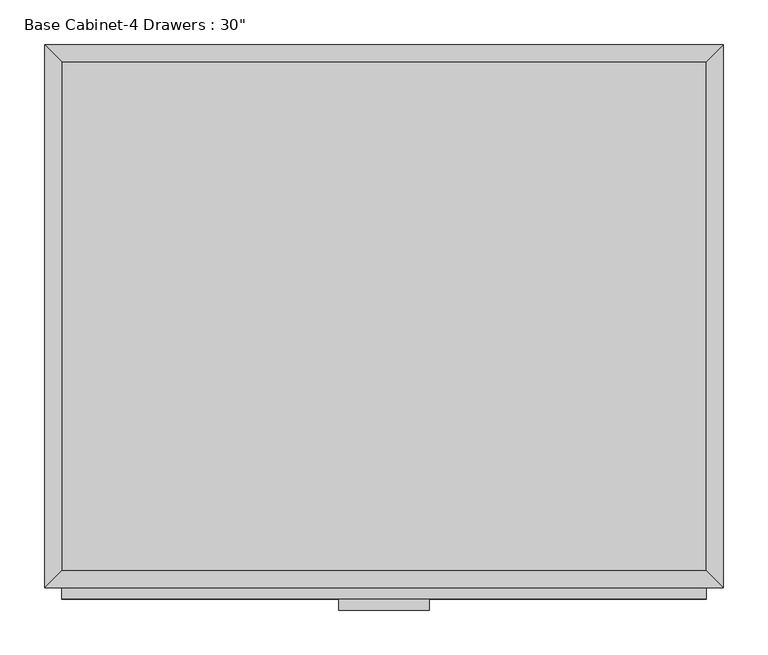
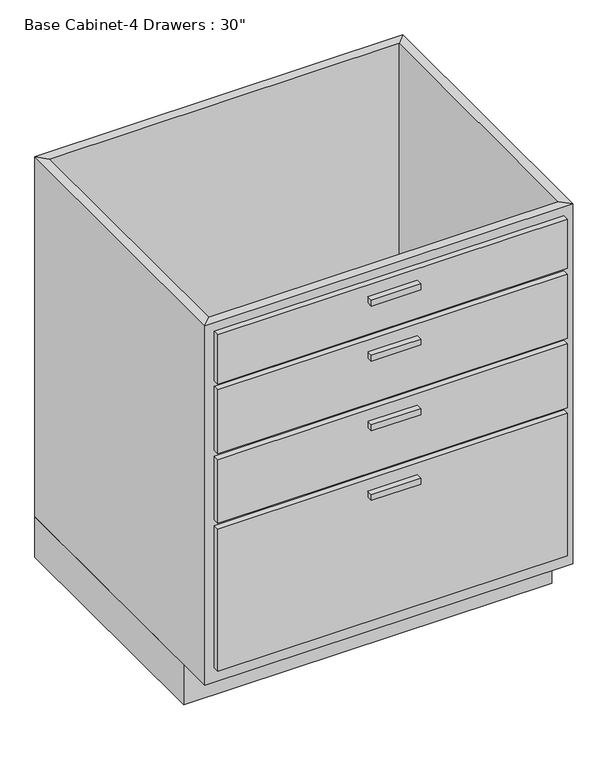
"""IFC4 building model written with IfcOpenShell, lengths in millimetres: furniture geometry."""

from ifc_helpers import new_model, si_unit, frame, origin, origin_with_axes, place, context, project, spatial, polyline, outline, extrude, faceted_brep, source, transform, mapped, element, save


def furniture_2c6c3b69(model_context):
    return source(origin(), model_context, "Body", "SolidModel", [
        extrude(outline(polyline([(69.5377049, -635.0), (-32.0622951, -635.0), (-32.0622951, -622.3), (69.5377049, -622.3), (69.5377049, -635.0)])), frame((0.0, 0.0, 819.15), z_axis=(0.0, 0.0, 1.0), x_axis=(1.0, 0.0, 0.0)), (0.0, 0.0, 1.0), 12.7),
        extrude(outline(polyline([(69.5377049, -635.0), (-32.0622951, -635.0), (-32.0622951, -622.3), (69.5377049, -622.3), (69.5377049, -635.0)])), frame((0.0, 0.0, 698.5), z_axis=(0.0, 0.0, 1.0), x_axis=(1.0, 0.0, 0.0)), (0.0, 0.0, 1.0), 12.7),
        extrude(outline(polyline([(69.5377049, -635.0), (-32.0622951, -635.0), (-32.0622951, -622.3), (69.5377049, -622.3), (69.5377049, -635.0)])), frame((0.0, 0.0, 546.1), z_axis=(0.0, 0.0, 1.0), x_axis=(1.0, 0.0, 0.0)), (0.0, 0.0, 1.0), 12.7),
        extrude(outline(polyline([(69.5377049, -635.0), (-32.0622951, -635.0), (-32.0622951, -622.3), (69.5377049, -622.3), (69.5377049, -635.0)])), frame((0.0, 0.0, 393.7), z_axis=(0.0, 0.0, 1.0), x_axis=(1.0, 0.0, 0.0)), (0.0, 0.0, 1.0), 12.7),
        extrude(outline(polyline([(380.6877049, -622.3), (-343.2122951, -622.3), (-343.2122951, -609.6), (380.6877049, -609.6), (380.6877049, -622.3)])), frame((0.0, 0.0, 749.3), z_axis=(0.0, 0.0, 1.0), x_axis=(1.0, 0.0, 0.0)), (0.0, 0.0, 1.0), 107.95),
        extrude(outline(polyline([(380.6877049, -622.3), (-343.2122951, -622.3), (-343.2122951, -609.6), (380.6877049, -609.6), (380.6877049, -622.3)])), frame((0.0, 0.0, 596.9), z_axis=(0.0, 0.0, 1.0), x_axis=(1.0, 0.0, 0.0)), (0.0, 0.0, 1.0), 139.7),
        extrude(outline(polyline([(380.6877049, -622.3), (-343.2122951, -622.3), (-343.2122951, -609.6), (380.6877049, -609.6), (380.6877049, -622.3)])), frame((0.0, 0.0, 444.5), z_axis=(0.0, 0.0, 1.0), x_axis=(1.0, 0.0, 0.0)), (0.0, 0.0, 1.0), 139.7),
        extrude(outline(polyline([(380.6877049, -622.3), (-343.2122951, -622.3), (-343.2122951, -609.6), (380.6877049, -609.6), (380.6877049, -622.3)])), frame((0.0, 0.0, 120.65), z_axis=(0.0, 0.0, 1.0), x_axis=(1.0, 0.0, 0.0)), (0.0, 0.0, 1.0), 311.15),
        extrude(outline(polyline([(380.6877049, -19.05), (380.6877049, -590.55), (-343.2122951, -590.55), (-343.2122951, -19.05), (380.6877049, -19.05)])), frame((0.0, 0.0, 88.9), z_axis=(0.0, 0.0, 1.0), x_axis=(1.0, 0.0, 0.0)), (0.0, 0.0, 1.0), 19.05),
        faceted_brep([(380.6877049, -590.55, 876.3), (380.6877049, -590.55, 88.9), (-343.2122951, -590.55, 88.9), (-343.2122951, -590.55, 876.3), (399.7377049, -609.6, 876.3), (-362.2622951, -609.6, 876.3), (399.7377049, -609.6, 88.9), (-362.2622951, -609.6, 88.9), (-343.2122951, -19.05, 88.9), (-343.2122951, -19.05, 876.3), (-362.2622951, 0.0, 876.3), (-362.2622951, 0.0, 88.9), (380.6877049, -19.05, 88.9), (380.6877049, -19.05, 876.3), (399.7377049, 0.0, 876.3), (399.7377049, 0.0, 88.9)], [[[0, 1, 2, 3]], [[4, 0, 3, 5]], [[6, 4, 5, 7]], [[1, 6, 7, 2]], [[3, 2, 8, 9]], [[5, 3, 9, 10]], [[7, 5, 10, 11]], [[2, 7, 11, 8]], [[9, 8, 12, 13]], [[10, 9, 13, 14]], [[11, 10, 14, 15]], [[8, 11, 15, 12]], [[13, 12, 1, 0]], [[14, 13, 0, 4]], [[15, 14, 4, 6]], [[12, 15, 6, 1]]]),
        extrude(outline(polyline([(399.7377049, 0.0), (399.7377049, -533.4), (-362.2622951, -533.4), (-362.2622951, 0.0), (399.7377049, 0.0)])), origin_with_axes(), (0.0, 0.0, 1.0), 88.9),
    ])


if __name__ == "__main__":
    model = new_model("IFC4")
    model_context = context("Model", 3, world=origin())
    ifc_project = project(units=[si_unit("LENGTHUNIT", "METRE", prefix="MILLI")], contexts=[model_context])
    site = spatial("IfcSite", under=ifc_project)
    building = spatial("IfcBuilding", under=site)
    placement = place(None, origin())
    furniture_shape = furniture_2c6c3b69(model_context)
    element("IfcFurniture", 1, ObjectType="Base Cabinet-4 Drawers : 30\"", at=placement, inside=building, context=model_context, shape_type="MappedRepresentation", body=[
        mapped(furniture_shape, transform((0.0, 0.0, 0.0), x_axis=(1.0, 0.0, 0.0), y_axis=(0.0, 1.0, 0.0), z_axis=(0.0, 0.0, 1.0))),
    ])
    save(model, "model.ifc")

# Revit data of these elements
# Type "Base Cabinet-4 Drawers : 30\""
#   COBie.Type.CreatedBy = "doug.wood@us.ibm.com"
#   COBie.Type.CreatedOn = "2016-04-14T02:14:45"
#   COBie.Type.Name = "Casework_Base Cabinet-4 Drawers_30\""
#   COBie.Type.Category = "23-40 35 17 47 11 : Kitchen Casework"
#   COBie.Type.Description = "Base Cabinet-4 Drawers_30\""
#   COBie.Type.Manufacturer = ""
#   COBie.Type.ModelNumber = ""
#   Assembly Code = "C1030410"
#   COBie.Type.ReplacementCost = 0
#   Depth = 2' - 0"
#   Height = 2' - 10 1/2"
#   Toe Depth = 0' - 3"
#   Toe Height = 0' - 3 1/2"
#   Width = 2' - 6"
#   COBie.Type = no
#   Cabinet Material = none
#   Door/Drawer Material = Cabinets
#   Handle Material = none
# Element 1 (IfcFurniture, "Base Cabinet-4 Drawers : 30\"")
#   Materials on its faces: "Cabinets"
# Materials
#   "Cabinets": class "Miscellaneous", colour RGB 249 249 249, transparency 0
